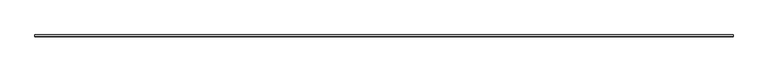
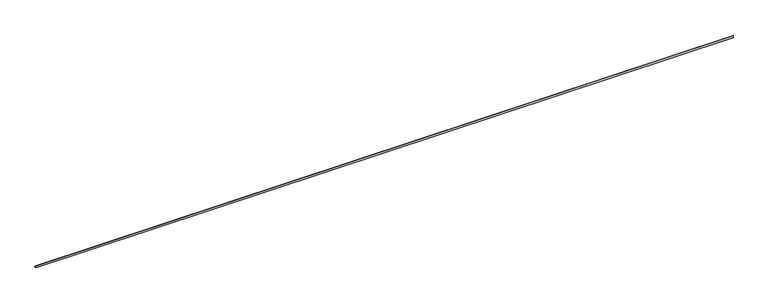
"""IFC4 building model written with IfcOpenShell, lengths in millimetres: proxy geometry, Stephan Brady4 : Stephan Brady."""

from ifc_helpers import new_model, si_unit, frame, origin, place, context, project, spatial, polyline, outline, extrude, source, transform, mapped, element, save


def generic_models_fd60ae16(model_context):
    return source(origin(), model_context, "Body", "SweptSolid", [
        extrude(outline(polyline([(-3327.5948735, 3226.308), (-3321.2448735, 3226.308), (-3308.5448735, 3213.608), (-3308.5448735, 3207.258), (-3327.5948735, 3207.258), (-3327.5948735, 3226.308)])), frame((-9238.6460766, 0.0, 0.0), z_axis=(1.0, 0.0, 0.0), x_axis=(0.0, 1.0, 0.0)), (0.0, 0.0, 1.0), 7443.2191995),
    ])


if __name__ == "__main__":
    model = new_model("IFC4")
    model_context = context("Model", 3, world=origin())
    ifc_project = project(units=[si_unit("LENGTHUNIT", "METRE", prefix="MILLI")], contexts=[model_context])
    site = spatial("IfcSite", under=ifc_project)
    building = spatial("IfcBuilding", under=site)
    placement = place(None, origin())
    generic_models_shape = generic_models_fd60ae16(model_context)
    element("IfcBuildingElementProxy", 1, Name="Stephan Brady4 : Stephan Brady", ObjectType="Stephan Brady4 : Stephan Brady", at=placement, inside=building, context=model_context, shape_type="MappedRepresentation", body=[
        mapped(generic_models_shape, transform((0.0, 0.0, 0.0), x_axis=(1.0, 0.0, 0.0), y_axis=(0.0, 1.0, 0.0), z_axis=(0.0, 0.0, 1.0))),
    ])
    save(model, "model.ifc")

# Revit data of these elements
# Element 1 (IfcBuildingElementProxy, "Stephan Brady4 : Stephan Brady")
#   Materials on its faces: "Aluminum"
# Materials
#   "Aluminum": class "Metal", colour RGB 247 247 247, transparency 0, Description = "Aluminum 6061", Cost = 0
